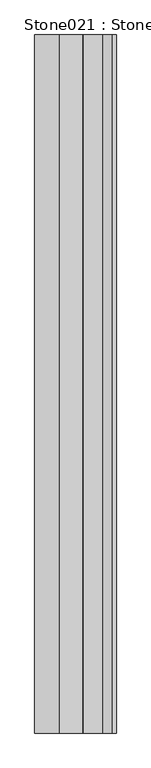
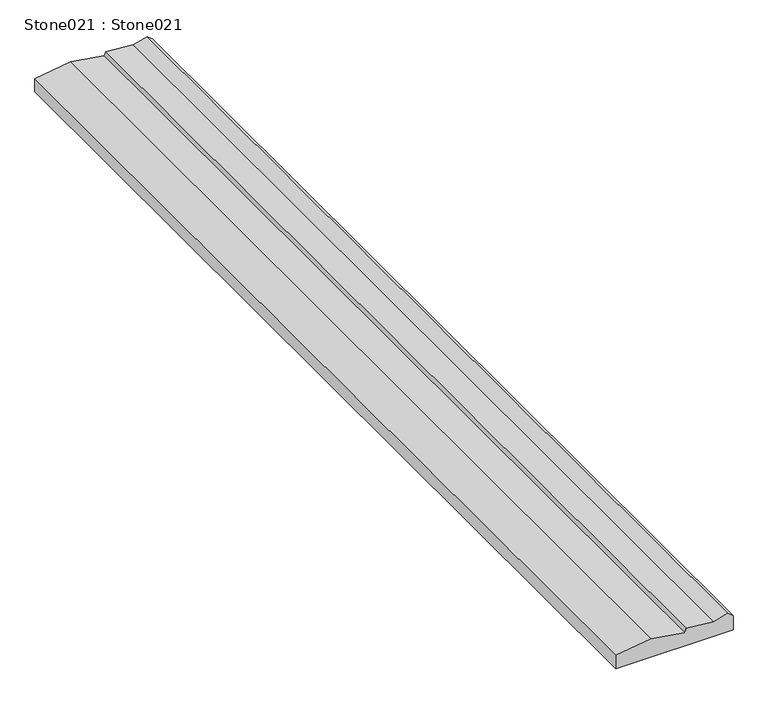
"""IFC4 building model written with IfcOpenShell, lengths in millimetres: proxy geometry, Stone021 : Stone021."""

from ifc_helpers import new_model, si_unit, frame, origin, place, context, project, spatial, polyline, outline, extrude, source, transform, mapped, element, save


def stone021_stone021_57c5fcad(model_context):
    return source(origin(), model_context, "Body", "SweptSolid", [
        extrude(outline(polyline([(33434.0234375, -10084.1142578), (33442.2773437, -10094.7001953), (33434.5546875, -10122.3896484), (33439.8789062, -10177.5029297), (33431.8945312, -10179.8994141), (33442.2773437, -10246.7275391), (33432.1601562, -10317.9149124), (33404.46875, -10317.9149124), (33404.46875, -10084.1142578), (33434.0234375, -10084.1142578)])), frame((0.0, 7982.1531721, 0.0), z_axis=(0.0, 1.0, 0.0), x_axis=(0.0, 0.0, 1.0)), (0.0, 0.0, 1.0), 2000.0),
    ])


if __name__ == "__main__":
    model = new_model("IFC4")
    model_context = context("Model", 3, world=origin())
    ifc_project = project(units=[si_unit("LENGTHUNIT", "METRE", prefix="MILLI")], contexts=[model_context])
    site = spatial("IfcSite", under=ifc_project)
    building = spatial("IfcBuilding", under=site)
    placement = place(None, origin())
    stone021_stone021_shape = stone021_stone021_57c5fcad(model_context)
    element("IfcBuildingElementProxy", 1, Name="Stone021 : Stone021", ObjectType="Stone021 : Stone021", at=placement, inside=building, context=model_context, shape_type="MappedRepresentation", body=[
        mapped(stone021_stone021_shape, transform((0.0, 0.0, 0.0), x_axis=(1.0, 0.0, 0.0), y_axis=(0.0, 1.0, 0.0), z_axis=(0.0, 0.0, 1.0))),
    ])
    save(model, "model.ifc")

# Revit data of these elements
# Type "Stone021 : Stone021"
#   NameOverride = "Stone021"
# Element 1 (IfcBuildingElementProxy, "Stone021 : Stone021")
#   Materials on its faces: "SPLIT FACE STONE 1032"
# Materials
#   "SPLIT FACE STONE 1032": class "Unassigned", colour RGB 205 195 181, transparency 0
